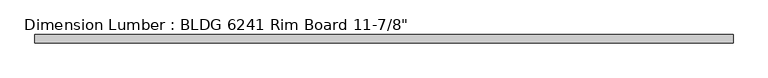
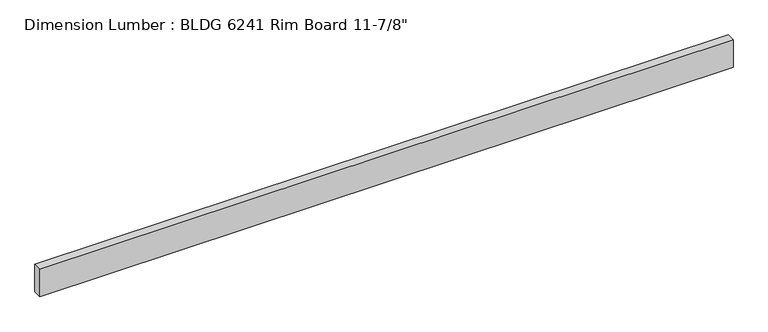
"""IFC4 building model written with IfcOpenShell, lengths in millimetres: beam geometry."""

from ifc_helpers import new_model, si_unit, frame, origin, place, context, project, spatial, polyline, outline, extrude, source, transform, mapped, element, save


def beam_45e17afb(model_context):
    return source(origin(), model_context, "Body", "SweptSolid", [
        extrude(outline(polyline([(3568.7, 44.45), (3568.7, -44.45), (-3657.6, -44.45), (-3657.6, 44.45), (3568.7, 44.45)])), frame((0.0, 0.0, -150.8125), z_axis=(0.0, 0.0, 1.0), x_axis=(1.0, 0.0, 0.0)), (0.0, 0.0, 1.0), 301.625),
    ])


if __name__ == "__main__":
    model = new_model("IFC4")
    model_context = context("Model", 3, world=origin())
    ifc_project = project(units=[si_unit("LENGTHUNIT", "METRE", prefix="MILLI")], contexts=[model_context])
    site = spatial("IfcSite", under=ifc_project)
    building = spatial("IfcBuilding", under=site)
    placement = place(None, origin())
    beam_shape = beam_45e17afb(model_context)
    element("IfcBeam", 1, ObjectType="Dimension Lumber : BLDG 6241 Rim Board 11-7/8\"", at=placement, inside=building, context=model_context, shape_type="MappedRepresentation", body=[
        mapped(beam_shape, transform((0.0, 0.0, 0.0), x_axis=(1.0, 0.0, 0.0), y_axis=(0.0, 1.0, 0.0), z_axis=(0.0, 0.0, 1.0))),
    ])
    save(model, "model.ifc")

# Revit data of these elements
# Type "Dimension Lumber : BLDG 6241 Rim Board 11-7/8\""
#   Assembly Code = "B10"
#   A = 0.273472 SF
#   Length [instance default] = 5' - 0"
#   b = 0' - 3 1/2"
#   d = 0' - 11 7/8"
#   Structural Material [instance default] = Softwood, Lumber
# Element 1 (IfcBeam, "Dimension Lumber : BLDG 6241 Rim Board 11-7/8\"")
#   Materials on its faces: "Softwood, Lumber"
# Materials
#   "Softwood, Lumber": class "Wood", colour RGB 223 192 134, transparency 0, Description = "Pinus Echinata", Cost = 0
